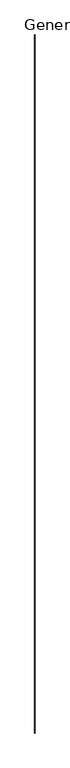
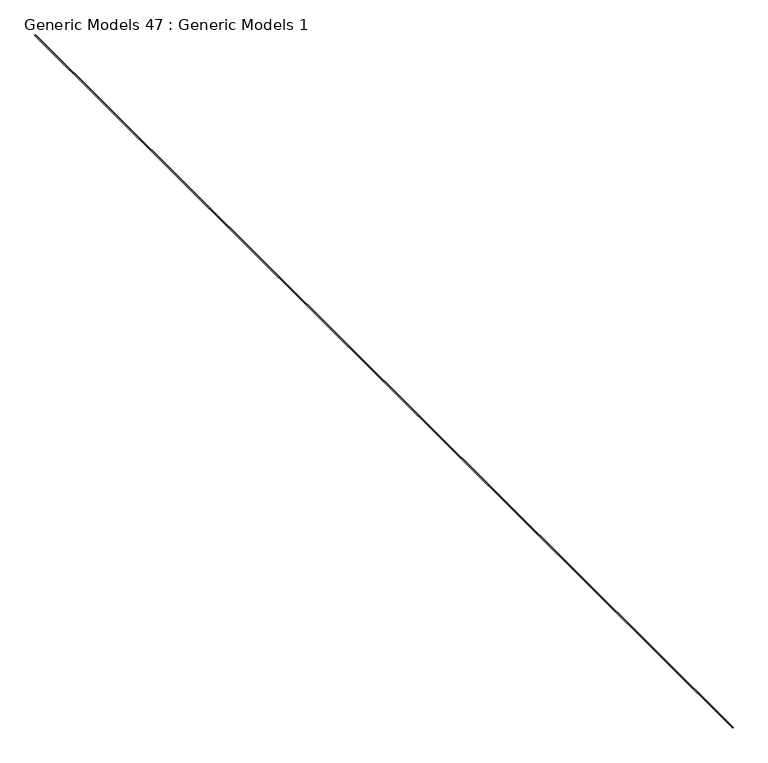
"""IFC4 building model written with IfcOpenShell, lengths in millimetres: proxy geometry, Generic Models 47 : Generic Models 1."""

from ifc_helpers import new_model, si_unit, point, frame, origin, place, context, project, spatial, polyline, circle_curve, ellipse_curve, trimmed, source, transform, mapped, element, save
from ifc_brep_helpers import plane_surface, cylinder_surface, revolved_surface, extruded_surface, advanced_brep


def generic_models_47_generic_models_1_faf58e0f(model_context):
    return source(origin(), model_context, "Body", "AdvancedBrep", [
        advanced_brep(
        [(32147.5090778, 25672.1156612, 266423.0271013), (32144.3340778, 25672.1156612, 266423.0271013), (32143.3823185, 25672.1156612, 266421.7564428), (32143.3823185, 25672.1156612, 266417.9477599), (32144.3340778, 25672.1156612, 266416.6771013), (32147.5090778, 25672.1156612, 266416.6771013), (32147.5090778, 40827.6606612, 266423.0271013), (32147.5090778, 40827.6606612, 266416.6771013), (32144.3340778, 40827.6606612, 266416.6771013), (32143.3823185, 40827.6606612, 266417.9477599), (32143.3823185, 40827.6606612, 266421.7564428), (32144.3340778, 40827.6606612, 266423.0271013)],
        [
            (0, 1),
            (1, 2, circle_curve(frame((32147.2488183, 25672.1156612, 266419.8521013), z_axis=(0.0, -1.0, 0.0), x_axis=(0.0, 0.0, 1.0)), 4.3100275)),
            (2, 3, ellipse_curve(frame((32139.5715778, 25672.1156612, 266419.8521013), z_axis=(0.0, -1.0, 0.0), x_axis=(1.0, 0.0, 0.0)), 4.7625, 3.175)),
            (3, 4, circle_curve(frame((32147.2488183, 25672.1156612, 266419.8521013), z_axis=(0.0, -1.0, 0.0), x_axis=(0.0, 0.0, 1.0)), 4.3100275)),
            (4, 5),
            (5, 0, circle_curve(frame((32150.4238183, 25672.1156612, 266419.8521013), z_axis=(0.0, 1.0, 0.0), x_axis=(0.0, 0.0, 1.0)), 4.3100275)),
            (6, 7, circle_curve(frame((32150.4238183, 40827.6606612, 266419.8521013), z_axis=(0.0, -1.0, 0.0), x_axis=(0.0, 0.0, 1.0)), 4.3100275)),
            (7, 8),
            (8, 9, circle_curve(frame((32147.2488183, 40827.6606612, 266419.8521013), z_axis=(0.0, 1.0, 0.0), x_axis=(0.0, 0.0, 1.0)), 4.3100275)),
            (9, 10, ellipse_curve(frame((32139.5715778, 40827.6606612, 266419.8521013), z_axis=(0.0, 1.0, 0.0), x_axis=(1.0, 0.0, 0.0)), 4.7625, 3.175)),
            (10, 11, circle_curve(frame((32147.2488183, 40827.6606612, 266419.8521013), z_axis=(0.0, 1.0, 0.0), x_axis=(0.0, 0.0, 1.0)), 4.3100275)),
            (11, 6),
            (5, 7),
            (6, 0),
            (11, 1),
            (3, 9),
            (8, 4),
            (2, 10),
        ],
        [
            plane_surface(frame((32147.5090778, 25672.1156612, 266416.6771013), z_axis=(0.0, -1.0, 0.0), x_axis=(0.0, 0.0, 1.0))),
            plane_surface(frame((32147.5090778, 40827.6606612, 266416.6771013), z_axis=(0.0, 1.0, 0.0), x_axis=(0.0, 0.0, 1.0))),
            revolved_surface(polyline([(32150.4238183, 40827.6606612, 266424.1621288), (32150.4238183, 25672.1156612, 266424.1621288)]), (32150.4238183, 25672.1156612, 266419.8521013), (0.0, 1.0, 0.0)),
            plane_surface(frame((32147.5090778, 25672.1156612, 266423.0271013), z_axis=(0.0, 0.0, 1.0), x_axis=(0.0, 1.0, 0.0))),
            cylinder_surface(frame((32147.2488183, 25672.1156612, 266419.8521013), z_axis=(0.0, -1.0, 0.0), x_axis=(0.0, 0.0, 1.0)), 4.3100275),
            plane_surface(frame((32144.3340778, 25672.1156612, 266416.6771013), z_axis=(0.0, 0.0, -1.0), x_axis=(0.0, 1.0, 0.0))),
            extruded_surface(trimmed(ellipse_curve(frame((32139.5715778, 40827.6606612, 266419.8521013), z_axis=(0.0, -1.0, 0.0), x_axis=(1.0, 0.0, 0.0)), 4.7625, 3.175), [point((32143.3823185, 40827.6606612, 266421.7564428))], [point((32143.3823185, 40827.6606612, 266417.9477599))], True, "CARTESIAN"), (0.0, -15155.545000000002, 0.0), 15155.545000000002),
        ],
        [
            (0, [[1, 2, 3, 4, 5, 6]]),
            (1, [[7, 8, 9, 10, 11, 12]]),
            (2, [[-6, 13, -7, 14]]),
            (3, [[-1, -14, -12, 15]]),
            (4, [[-4, 16, -9, 17]]),
            (5, [[-5, -17, -8, -13]]),
            (6, [[-3, 18, -10, -16]]),
            (4, [[-2, -15, -11, -18]]),
        ],
    ),
    ])


if __name__ == "__main__":
    model = new_model("IFC4")
    model_context = context("Model", 3, world=origin())
    ifc_project = project(units=[si_unit("LENGTHUNIT", "METRE", prefix="MILLI")], contexts=[model_context])
    site = spatial("IfcSite", under=ifc_project)
    building = spatial("IfcBuilding", under=site)
    placement = place(None, origin())
    generic_models_47_generic_models_1_shape = generic_models_47_generic_models_1_faf58e0f(model_context)
    element("IfcBuildingElementProxy", 1, Name="Generic Models 47 : Generic Models 1", ObjectType="Generic Models 47 : Generic Models 1", at=placement, inside=building, context=model_context, shape_type="MappedRepresentation", body=[
        mapped(generic_models_47_generic_models_1_shape, transform((0.0, 0.0, 0.0), x_axis=(1.0, 0.0, 0.0), y_axis=(0.0, 1.0, 0.0), z_axis=(0.0, 0.0, 1.0))),
    ])
    save(model, "model.ifc")

# Revit data of these elements
# Element 1 (IfcBuildingElementProxy, "Generic Models 47 : Generic Models 1")
#   Materials on its faces: "SEALANT (& BACKER ROD IF NECESSARY)"
# Materials
#   "SEALANT (& BACKER ROD IF NECESSARY)": class "Generic", colour RGB 176 213 108, transparency 0, Cost = 0
